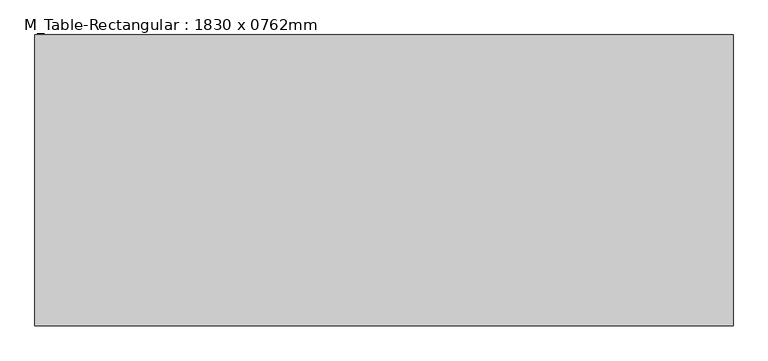
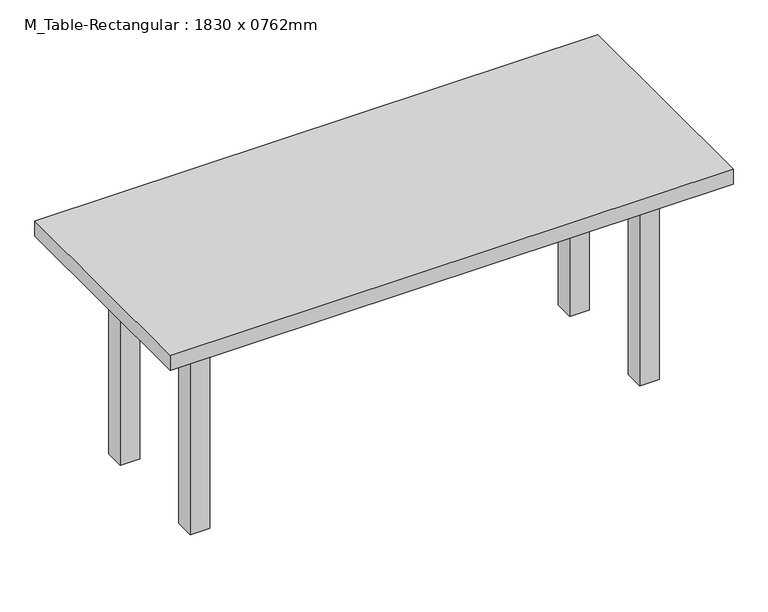
"""IFC4 building model written with IfcOpenShell, lengths in millimetres: furniture geometry, M_Table-Rectangular : 1830 x 0762mm."""

import ifcopenshell
import ifcopenshell.guid

model = None  # the IFC model being written
_history = None  # IfcOwnerHistory: only IFC2X3 demands one
_inside = {}  # id of a spatial element -> (the spatial element, [elements in it])
_under = {}  # id of a project, library or spatial element -> (it, [spatial elements below it])
_declared = {}  # id of a project -> (the project, [libraries it declares])
_typed = {}  # id of a type object -> (the type object, [elements of that type])
_made_of = {}  # id of a material, layer set ... -> (it, [elements and type objects made of it])


def new_model(schema):
    """Start an empty IFC model of exactly this schema.

    Asked for "IFC4X3", IfcOpenShell would pick the latest addendum, in which some entities
    have other attributes; the version numbers below select the first issue.
    IFC2X3 requires an IfcOwnerHistory on every rooted entity: one is made here for all.
    """
    global model, _history
    if schema == "IFC4X3":
        model = ifcopenshell.file(schema_version=(4, 3, 0, 0))
    else:
        model = ifcopenshell.file(schema=schema)
    _inside.clear()
    _under.clear()
    _declared.clear()
    _typed.clear()
    _made_of.clear()
    _history = None
    if model.schema == "IFC2X3":
        org = make("IfcOrganization", Name="unknown")
        user = make(
            "IfcPersonAndOrganization",
            ThePerson=make("IfcPerson", FamilyName="unknown"),
            TheOrganization=org,
        )
        app = make(
            "IfcApplication",
            ApplicationDeveloper=org,
            Version="unknown",
            ApplicationFullName="unknown",
            ApplicationIdentifier="unknown",
        )
        _history = make(
            "IfcOwnerHistory",
            OwningUser=user,
            OwningApplication=app,
            ChangeAction="ADDED",
            CreationDate=0,
        )
    return model


def make(cls, **values):
    """One entity of the class cls with the attributes given. An attribute that is None is left unset."""
    return model.create_entity(
        cls, **{name: value for name, value in values.items() if value is not None}
    )


def rooted(cls, **values):
    """An entity with a GlobalId (a new one), such as an element, a storey or a relation."""
    return make(cls, GlobalId=ifcopenshell.guid.new(), OwnerHistory=_history, **values)


def si_unit(unit_type, name, prefix=None):
    """IfcSIUnit, for example si_unit("LENGTHUNIT", "METRE", prefix="MILLI")."""
    return make("IfcSIUnit", UnitType=unit_type, Prefix=prefix, Name=name)


def assignment(units):
    """IfcUnitAssignment: the units of a project."""
    return None if units is None else make("IfcUnitAssignment", Units=units)


def point(xyz):
    """IfcCartesianPoint."""
    return None if xyz is None else make("IfcCartesianPoint", Coordinates=xyz)


def direction(xyz):
    """IfcDirection."""
    return None if xyz is None else make("IfcDirection", DirectionRatios=xyz)


def frame(location, z_axis=None, x_axis=None):
    """IfcAxis2Placement3D, a coordinate frame: its origin and axes. An axis left out is left unset."""
    return make(
        "IfcAxis2Placement3D",
        Location=point(location),
        Axis=direction(z_axis),
        RefDirection=direction(x_axis),
    )


def origin():
    """The frame at (0, 0, 0) with its axes left unset."""
    return frame((0.0, 0.0, 0.0))


def origin_with_axes():
    """The frame at (0, 0, 0) with the z axis (0, 0, 1) and the x axis (1, 0, 0) written out."""
    return frame((0.0, 0.0, 0.0), z_axis=(0.0, 0.0, 1.0), x_axis=(1.0, 0.0, 0.0))


def place(relative_to, where):
    """IfcLocalPlacement: puts the frame where relative to a parent placement (None: the world)."""
    return make(
        "IfcLocalPlacement", PlacementRelTo=relative_to, RelativePlacement=where
    )


def context(
    kind, dimensions, precision=None, world=None, true_north=None, identifier=None
):
    """IfcGeometricRepresentationContext, for example the 3D "Model" context."""
    return make(
        "IfcGeometricRepresentationContext",
        ContextIdentifier=identifier,
        ContextType=kind,
        CoordinateSpaceDimension=dimensions,
        Precision=precision,
        WorldCoordinateSystem=world,
        TrueNorth=true_north,
    )


def project(units=None, contexts=None):
    """IfcProject with its units and contexts."""
    return rooted(
        "IfcProject",
        Name="project",
        RepresentationContexts=contexts,
        UnitsInContext=assignment(units),
    )


def spatial(cls, under=None, at=None, **own):
    """A site, building, storey or space (cls), placed at a placement, below another one or the project."""
    s = rooted(cls, ObjectPlacement=at, **own)
    if under is not None:
        _under.setdefault(under.id(), (under, []))[1].append(s)
    return s


def polyline(points):
    """IfcPolyline through the points."""
    return make("IfcPolyline", Points=[point(p) for p in points])


def outline(outer, holes=None, kind="AREA"):
    """IfcArbitraryClosedProfileDef: a profile drawn as a closed curve; with holes, ...WithVoids."""
    if holes is None:
        return make("IfcArbitraryClosedProfileDef", ProfileType=kind, OuterCurve=outer)
    return make(
        "IfcArbitraryProfileDefWithVoids",
        ProfileType=kind,
        OuterCurve=outer,
        InnerCurves=holes,
    )


def extrude(swept, where, along, depth):
    """IfcExtrudedAreaSolid: the profile swept, set in the frame where, extruded along a direction by depth."""
    return make(
        "IfcExtrudedAreaSolid",
        SweptArea=swept,
        Position=where,
        ExtrudedDirection=direction(along),
        Depth=depth,
    )


def shape(context_of_items, identifier, shape_type, items):
    """IfcShapeRepresentation: the items that make up one representation, for example the "Body"."""
    return make(
        "IfcShapeRepresentation",
        ContextOfItems=context_of_items,
        RepresentationIdentifier=identifier,
        RepresentationType=shape_type,
        Items=items,
    )


def source(mapping_origin, context_of_items, identifier, shape_type, items):
    """IfcRepresentationMap: a shape defined once, which mapped items show again and again."""
    return make(
        "IfcRepresentationMap",
        MappingOrigin=mapping_origin,
        MappedRepresentation=shape(context_of_items, identifier, shape_type, items),
    )


def transform(
    local_origin,
    x_axis=None,
    y_axis=None,
    z_axis=None,
    scale=None,
    scale2=None,
    scale3=None,
    uniform=True,
):
    """IfcCartesianTransformationOperator3D, or its non-uniform kind. x_axis, y_axis, z_axis: its Axis1, 2, 3."""
    if uniform:
        return make(
            "IfcCartesianTransformationOperator3D",
            Axis1=direction(x_axis),
            Axis2=direction(y_axis),
            LocalOrigin=point(local_origin),
            Scale=scale,
            Axis3=direction(z_axis),
        )
    return make(
        "IfcCartesianTransformationOperator3DnonUniform",
        Axis1=direction(x_axis),
        Axis2=direction(y_axis),
        LocalOrigin=point(local_origin),
        Scale=scale,
        Axis3=direction(z_axis),
        Scale2=scale2,
        Scale3=scale3,
    )


def mapped(mapping_source, mapping_target):
    """IfcMappedItem: shows the shape of a source again, moved by a transform."""
    return make(
        "IfcMappedItem", MappingSource=mapping_source, MappingTarget=mapping_target
    )


def made_of(thing, what):
    """Note that an element or type object is made of a material, layer set ...; save() writes the relation."""
    if what is not None:
        _made_of.setdefault(what.id(), (what, []))[1].append(thing)
    return thing


def element(
    cls,
    number,
    at=None,
    inside=None,
    cuts=None,
    type_object=None,
    material=None,
    context=None,
    identifier="Body",
    shape_type=None,
    held_by="IfcProductDefinitionShape",
    body=None,
    shapes=None,
    **own,
):
    """One element of the class cls, such as IfcWall. Its Tag is "e" and its number.

    at: its placement. inside: the storey or other place that contains it. cuts: it is an
    opening in that element (IfcRelVoidsElement). A single representation is given by context,
    identifier, shape_type and body (its items); several are given by shapes. held_by: the class
    of the entity that holds the representations. save() writes the other relations.
    """
    e = rooted(cls, Tag="e%d" % number, ObjectPlacement=at, **own)
    if body is not None:
        shapes = [shape(context, identifier, shape_type, body)]
    if shapes is not None:
        e.Representation = make(held_by, Representations=shapes)
    if inside is not None:
        _inside.setdefault(inside.id(), (inside, []))[1].append(e)
    if cuts is not None:
        rooted(
            "IfcRelVoidsElement", RelatingBuildingElement=cuts, RelatedOpeningElement=e
        )
    if type_object is not None:
        _typed.setdefault(type_object.id(), (type_object, []))[1].append(e)
    return made_of(e, material)


def aggregate(whole, parts):
    """IfcRelAggregates: a whole, such as a stair, and the parts it consists of."""
    return rooted("IfcRelAggregates", RelatingObject=whole, RelatedObjects=parts)


def save(model, path):
    """Write the relations noted so far, then the file.

    IfcRelAggregates (storeys below a building ...), IfcRelContainedInSpatialStructure (elements
    in a storey), IfcRelDefinesByType, IfcRelAssociatesMaterial and IfcRelDeclares: one each for
    every whole, place, type object, material and project.
    """
    for whole, parts in _under.values():
        aggregate(whole, parts)
    for where, things in _inside.values():
        rooted(
            "IfcRelContainedInSpatialStructure",
            RelatedElements=things,
            RelatingStructure=where,
        )
    for kind, things in _typed.values():
        rooted("IfcRelDefinesByType", RelatedObjects=things, RelatingType=kind)
    for what, things in _made_of.values():
        rooted("IfcRelAssociatesMaterial", RelatedObjects=things, RelatingMaterial=what)
    for by, libraries in _declared.values():
        rooted("IfcRelDeclares", RelatingContext=by, RelatedDefinitions=libraries)
    model.write(path)


def m_table_rectangular_1830_x_0762mm_a0b3b7a0(model_context):
    return source(origin(), model_context, "Body", "SweptSolid", [
        extrude(outline(polyline([(699.1, 190.5), (699.1, 165.1), (-699.1, 165.1), (-699.1, 190.5), (699.1, 190.5)])), frame((0.0, 0.0, 609.6), z_axis=(0.0, 0.0, 1.0), x_axis=(1.0, 0.0, 0.0)), (0.0, 0.0, 1.0), 101.6),
        extrude(outline(polyline([(699.1, -190.5), (-699.1, -190.5), (-699.1, -165.1), (699.1, -165.1), (699.1, -190.5)])), frame((0.0, 0.0, 609.6), z_axis=(0.0, 0.0, 1.0), x_axis=(1.0, 0.0, 0.0)), (0.0, 0.0, 1.0), 101.6),
        extrude(outline(polyline([(-711.8, -165.1), (-737.2, -165.1), (-737.2, 165.1), (-711.8, 165.1), (-711.8, -165.1)])), frame((0.0, 0.0, 609.6), z_axis=(0.0, 0.0, 1.0), x_axis=(1.0, 0.0, 0.0)), (0.0, 0.0, 1.0), 101.6),
        extrude(outline(polyline([(711.8, -165.1), (711.8, 165.1), (737.2, 165.1), (737.2, -165.1), (711.8, -165.1)])), frame((0.0, 0.0, 609.6), z_axis=(0.0, 0.0, 1.0), x_axis=(1.0, 0.0, 0.0)), (0.0, 0.0, 1.0), 101.6),
        extrude(outline(polyline([(915.0, 381.0), (915.0, -381.0), (-915.0, -381.0), (-915.0, 381.0), (915.0, 381.0)])), frame((0.0, 0.0, 711.2), z_axis=(0.0, 0.0, 1.0), x_axis=(1.0, 0.0, 0.0)), (0.0, 0.0, 1.0), 50.8),
        extrude(outline(polyline([(-699.1, 228.6), (-699.1, 165.1), (-762.6, 165.1), (-762.6, 228.6), (-699.1, 228.6)])), origin_with_axes(), (0.0, 0.0, 1.0), 711.2),
        extrude(outline(polyline([(699.1, 228.6), (762.6, 228.6), (762.6, 165.1), (699.1, 165.1), (699.1, 228.6)])), origin_with_axes(), (0.0, 0.0, 1.0), 711.2),
        extrude(outline(polyline([(-699.1, -228.6), (-762.6, -228.6), (-762.6, -165.1), (-699.1, -165.1), (-699.1, -228.6)])), origin_with_axes(), (0.0, 0.0, 1.0), 711.2),
        extrude(outline(polyline([(699.1, -228.6), (699.1, -165.1), (762.6, -165.1), (762.6, -228.6), (699.1, -228.6)])), origin_with_axes(), (0.0, 0.0, 1.0), 711.2),
    ])


if __name__ == "__main__":
    model = new_model("IFC4")
    model_context = context("Model", 3, world=origin())
    ifc_project = project(units=[si_unit("LENGTHUNIT", "METRE", prefix="MILLI")], contexts=[model_context])
    site = spatial("IfcSite", under=ifc_project)
    building = spatial("IfcBuilding", under=site)
    placement = place(None, origin())
    m_table_rectangular_1830_x_0762mm_shape = m_table_rectangular_1830_x_0762mm_a0b3b7a0(model_context)
    element("IfcFurniture", 1, ObjectType="M_Table-Rectangular : 1830 x 0762mm", at=placement, inside=building, context=model_context, shape_type="MappedRepresentation", body=[
        mapped(m_table_rectangular_1830_x_0762mm_shape, transform((0.0, 0.0, 0.0), x_axis=(1.0, 0.0, 0.0), y_axis=(0.0, 1.0, 0.0), z_axis=(0.0, 0.0, 1.0))),
    ])
    save(model, "model.ifc")

# Revit data of these elements
# Type "M_Table-Rectangular : 1830 x 0762mm"
#   Height = 762 mm
#   Length = 1830 mm
#   Width = 762 mm
#   Base Material = Birch
#   Top Material = Birch
#   Default Elevation = 0
# Element 1 (IfcFurniture, "M_Table-Rectangular : 1830 x 0762mm")
#   Materials on its faces: "Birch"
# Materials
#   "Birch": class "Wood", colour RGB 224 178 126, transparency 0, Description = "Betula Alleghaniensis", Cost = 0
